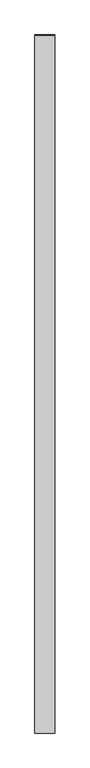
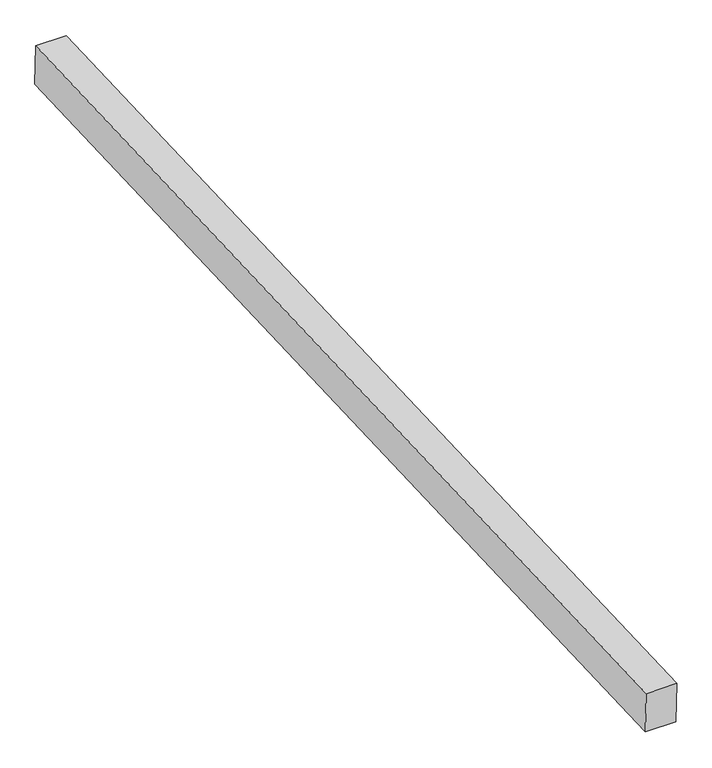
"""IFC4 building model written with IfcOpenShell, lengths in millimetres: proxy geometry, Generic Models 7:Generic Models 1:8:Generic Models 1:8 : Generic Models 7:Generic Models 1:337419:39 : Generic Models 7:Generic Models 1:8:Generic Models 1:8 : Generic Models 7:Generic Models 1:337419:315935."""

import ifcopenshell
import ifcopenshell.guid

model = None  # the IFC model being written
_history = None  # IfcOwnerHistory: only IFC2X3 demands one
_inside = {}  # id of a spatial element -> (the spatial element, [elements in it])
_under = {}  # id of a project, library or spatial element -> (it, [spatial elements below it])
_declared = {}  # id of a project -> (the project, [libraries it declares])
_typed = {}  # id of a type object -> (the type object, [elements of that type])
_made_of = {}  # id of a material, layer set ... -> (it, [elements and type objects made of it])


def new_model(schema):
    """Start an empty IFC model of exactly this schema.

    Asked for "IFC4X3", IfcOpenShell would pick the latest addendum, in which some entities
    have other attributes; the version numbers below select the first issue.
    IFC2X3 requires an IfcOwnerHistory on every rooted entity: one is made here for all.
    """
    global model, _history
    if schema == "IFC4X3":
        model = ifcopenshell.file(schema_version=(4, 3, 0, 0))
    else:
        model = ifcopenshell.file(schema=schema)
    _inside.clear()
    _under.clear()
    _declared.clear()
    _typed.clear()
    _made_of.clear()
    _history = None
    if model.schema == "IFC2X3":
        org = make("IfcOrganization", Name="unknown")
        user = make(
            "IfcPersonAndOrganization",
            ThePerson=make("IfcPerson", FamilyName="unknown"),
            TheOrganization=org,
        )
        app = make(
            "IfcApplication",
            ApplicationDeveloper=org,
            Version="unknown",
            ApplicationFullName="unknown",
            ApplicationIdentifier="unknown",
        )
        _history = make(
            "IfcOwnerHistory",
            OwningUser=user,
            OwningApplication=app,
            ChangeAction="ADDED",
            CreationDate=0,
        )
    return model


def make(cls, **values):
    """One entity of the class cls with the attributes given. An attribute that is None is left unset."""
    return model.create_entity(
        cls, **{name: value for name, value in values.items() if value is not None}
    )


def rooted(cls, **values):
    """An entity with a GlobalId (a new one), such as an element, a storey or a relation."""
    return make(cls, GlobalId=ifcopenshell.guid.new(), OwnerHistory=_history, **values)


def si_unit(unit_type, name, prefix=None):
    """IfcSIUnit, for example si_unit("LENGTHUNIT", "METRE", prefix="MILLI")."""
    return make("IfcSIUnit", UnitType=unit_type, Prefix=prefix, Name=name)


def assignment(units):
    """IfcUnitAssignment: the units of a project."""
    return None if units is None else make("IfcUnitAssignment", Units=units)


def point(xyz):
    """IfcCartesianPoint."""
    return None if xyz is None else make("IfcCartesianPoint", Coordinates=xyz)


def direction(xyz):
    """IfcDirection."""
    return None if xyz is None else make("IfcDirection", DirectionRatios=xyz)


def frame(location, z_axis=None, x_axis=None):
    """IfcAxis2Placement3D, a coordinate frame: its origin and axes. An axis left out is left unset."""
    return make(
        "IfcAxis2Placement3D",
        Location=point(location),
        Axis=direction(z_axis),
        RefDirection=direction(x_axis),
    )


def origin():
    """The frame at (0, 0, 0) with its axes left unset."""
    return frame((0.0, 0.0, 0.0))


def place(relative_to, where):
    """IfcLocalPlacement: puts the frame where relative to a parent placement (None: the world)."""
    return make(
        "IfcLocalPlacement", PlacementRelTo=relative_to, RelativePlacement=where
    )


def context(
    kind, dimensions, precision=None, world=None, true_north=None, identifier=None
):
    """IfcGeometricRepresentationContext, for example the 3D "Model" context."""
    return make(
        "IfcGeometricRepresentationContext",
        ContextIdentifier=identifier,
        ContextType=kind,
        CoordinateSpaceDimension=dimensions,
        Precision=precision,
        WorldCoordinateSystem=world,
        TrueNorth=true_north,
    )


def project(units=None, contexts=None):
    """IfcProject with its units and contexts."""
    return rooted(
        "IfcProject",
        Name="project",
        RepresentationContexts=contexts,
        UnitsInContext=assignment(units),
    )


def spatial(cls, under=None, at=None, **own):
    """A site, building, storey or space (cls), placed at a placement, below another one or the project."""
    s = rooted(cls, ObjectPlacement=at, **own)
    if under is not None:
        _under.setdefault(under.id(), (under, []))[1].append(s)
    return s


def polyline(points):
    """IfcPolyline through the points."""
    return make("IfcPolyline", Points=[point(p) for p in points])


def outline(outer, holes=None, kind="AREA"):
    """IfcArbitraryClosedProfileDef: a profile drawn as a closed curve; with holes, ...WithVoids."""
    if holes is None:
        return make("IfcArbitraryClosedProfileDef", ProfileType=kind, OuterCurve=outer)
    return make(
        "IfcArbitraryProfileDefWithVoids",
        ProfileType=kind,
        OuterCurve=outer,
        InnerCurves=holes,
    )


def extrude(swept, where, along, depth):
    """IfcExtrudedAreaSolid: the profile swept, set in the frame where, extruded along a direction by depth."""
    return make(
        "IfcExtrudedAreaSolid",
        SweptArea=swept,
        Position=where,
        ExtrudedDirection=direction(along),
        Depth=depth,
    )


def shape(context_of_items, identifier, shape_type, items):
    """IfcShapeRepresentation: the items that make up one representation, for example the "Body"."""
    return make(
        "IfcShapeRepresentation",
        ContextOfItems=context_of_items,
        RepresentationIdentifier=identifier,
        RepresentationType=shape_type,
        Items=items,
    )


def source(mapping_origin, context_of_items, identifier, shape_type, items):
    """IfcRepresentationMap: a shape defined once, which mapped items show again and again."""
    return make(
        "IfcRepresentationMap",
        MappingOrigin=mapping_origin,
        MappedRepresentation=shape(context_of_items, identifier, shape_type, items),
    )


def transform(
    local_origin,
    x_axis=None,
    y_axis=None,
    z_axis=None,
    scale=None,
    scale2=None,
    scale3=None,
    uniform=True,
):
    """IfcCartesianTransformationOperator3D, or its non-uniform kind. x_axis, y_axis, z_axis: its Axis1, 2, 3."""
    if uniform:
        return make(
            "IfcCartesianTransformationOperator3D",
            Axis1=direction(x_axis),
            Axis2=direction(y_axis),
            LocalOrigin=point(local_origin),
            Scale=scale,
            Axis3=direction(z_axis),
        )
    return make(
        "IfcCartesianTransformationOperator3DnonUniform",
        Axis1=direction(x_axis),
        Axis2=direction(y_axis),
        LocalOrigin=point(local_origin),
        Scale=scale,
        Axis3=direction(z_axis),
        Scale2=scale2,
        Scale3=scale3,
    )


def mapped(mapping_source, mapping_target):
    """IfcMappedItem: shows the shape of a source again, moved by a transform."""
    return make(
        "IfcMappedItem", MappingSource=mapping_source, MappingTarget=mapping_target
    )


def made_of(thing, what):
    """Note that an element or type object is made of a material, layer set ...; save() writes the relation."""
    if what is not None:
        _made_of.setdefault(what.id(), (what, []))[1].append(thing)
    return thing


def element(
    cls,
    number,
    at=None,
    inside=None,
    cuts=None,
    type_object=None,
    material=None,
    context=None,
    identifier="Body",
    shape_type=None,
    held_by="IfcProductDefinitionShape",
    body=None,
    shapes=None,
    **own,
):
    """One element of the class cls, such as IfcWall. Its Tag is "e" and its number.

    at: its placement. inside: the storey or other place that contains it. cuts: it is an
    opening in that element (IfcRelVoidsElement). A single representation is given by context,
    identifier, shape_type and body (its items); several are given by shapes. held_by: the class
    of the entity that holds the representations. save() writes the other relations.
    """
    e = rooted(cls, Tag="e%d" % number, ObjectPlacement=at, **own)
    if body is not None:
        shapes = [shape(context, identifier, shape_type, body)]
    if shapes is not None:
        e.Representation = make(held_by, Representations=shapes)
    if inside is not None:
        _inside.setdefault(inside.id(), (inside, []))[1].append(e)
    if cuts is not None:
        rooted(
            "IfcRelVoidsElement", RelatingBuildingElement=cuts, RelatedOpeningElement=e
        )
    if type_object is not None:
        _typed.setdefault(type_object.id(), (type_object, []))[1].append(e)
    return made_of(e, material)


def aggregate(whole, parts):
    """IfcRelAggregates: a whole, such as a stair, and the parts it consists of."""
    return rooted("IfcRelAggregates", RelatingObject=whole, RelatedObjects=parts)


def save(model, path):
    """Write the relations noted so far, then the file.

    IfcRelAggregates (storeys below a building ...), IfcRelContainedInSpatialStructure (elements
    in a storey), IfcRelDefinesByType, IfcRelAssociatesMaterial and IfcRelDeclares: one each for
    every whole, place, type object, material and project.
    """
    for whole, parts in _under.values():
        aggregate(whole, parts)
    for where, things in _inside.values():
        rooted(
            "IfcRelContainedInSpatialStructure",
            RelatedElements=things,
            RelatingStructure=where,
        )
    for kind, things in _typed.values():
        rooted("IfcRelDefinesByType", RelatedObjects=things, RelatingType=kind)
    for what, things in _made_of.values():
        rooted("IfcRelAssociatesMaterial", RelatedObjects=things, RelatingMaterial=what)
    for by, libraries in _declared.values():
        rooted("IfcRelDeclares", RelatingContext=by, RelatedDefinitions=libraries)
    model.write(path)


def generic_models_cd876d45(model_context):
    return source(origin(), model_context, "Body", "SweptSolid", [
        extrude(outline(polyline([(-581229.2495411, 3818.908703), (-576356.3266468, 4021.9471569), (-576348.7597251, 3831.5971524), (-581221.3189223, 3628.5738526), (-581229.2495411, 3818.908703)])), frame((663521.4117239, 0.0, 0.0), z_axis=(1.0, 0.0, 0.0), x_axis=(0.0, 1.0, 0.0)), (0.0, 0.0, 1.0), 139.7),
    ])


if __name__ == "__main__":
    model = new_model("IFC4")
    model_context = context("Model", 3, world=origin())
    ifc_project = project(units=[si_unit("LENGTHUNIT", "METRE", prefix="MILLI")], contexts=[model_context])
    site = spatial("IfcSite", under=ifc_project)
    building = spatial("IfcBuilding", under=site)
    placement = place(None, origin())
    generic_models_shape = generic_models_cd876d45(model_context)
    element("IfcBuildingElementProxy", 1, Name="Generic Models 7:Generic Models 1:8:Generic Models 1:8 : Generic Models 7:Generic Models 1:337419:39 : Generic Models 7:Generic Models 1:8:Generic Models 1:8 : Generic Models 7:Generic Models 1:337419:315935", ObjectType="Generic Models 7:Generic Models 1:8:Generic Models 1:8 : Generic Models 7:Generic Models 1:337419:39 : Generic Models 7:Generic Models 1:8:Generic Models 1:8 : Generic Models 7:Generic Models 1:337419:315935", at=placement, inside=building, context=model_context, shape_type="MappedRepresentation", body=[
        mapped(generic_models_shape, transform((0.0, 0.0, 0.0), x_axis=(1.0, 0.0, 0.0), y_axis=(0.0, 1.0, 0.0), z_axis=(0.0, 0.0, 1.0))),
    ])
    save(model, "model.ifc")

# Revit data of these elements
# Type "Generic Models 7:Generic Models 1:8:Generic Models 1:8 : Generic Models 7:Generic Models 1:337419:39 : Generic Models 7:Generic Models 1:8:Generic Models 1:8 : Generic Models 7:Generic Models 1:337419:315935"
#   NameOverride = "Generic Models 7:Generic Models 1:8:Generic Models 1:8 : Generic Models 7:Generic Models 1:337419:315935"
#   ObjectTypeOverride = "Generic Models 1:8 : Generic Models 7:Generic Models 1:337419"
#   Reference = "Generic Models 1"
#   Tag = "315935"
# Element 1 (IfcBuildingElementProxy, "Generic Models 7:Generic Models 1:8:Generic Models 1:8 : Generic Models 7:Generic Models 1:337419:39 : Generic Models 7:Generic Models 1:8:Generic Models 1:8 : Generic Models 7:Generic Models 1:337419:315935")
#   Materials on its faces: "5 1/2\" X 7 1/2\" EXTERIOR GRADE GLULAM BEAMS"
# Materials
#   "5 1/2\" X 7 1/2\" EXTERIOR GRADE GLULAM BEAMS": class "Wood", colour RGB 183 134 68, transparency 0, Keynote = "M06181300.01", Description = "Pinus Echinata", Cost = 0
